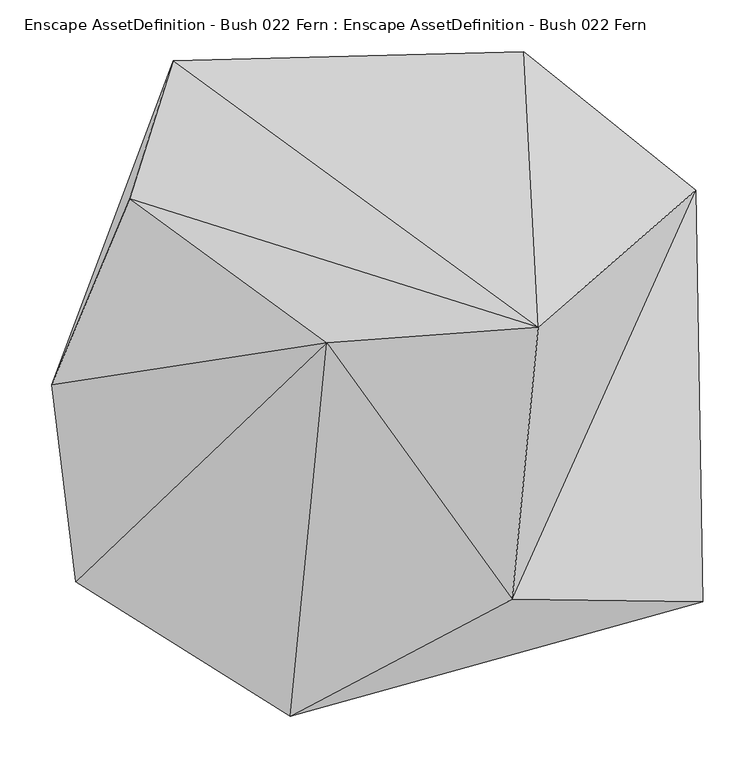
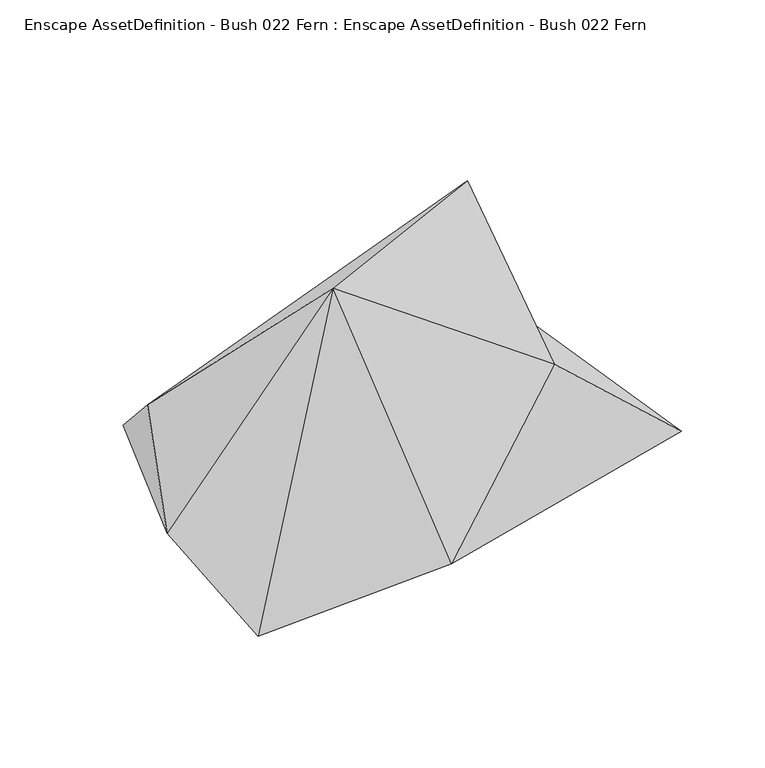
"""IFC4 building model written with IfcOpenShell, lengths in millimetres: geographic element geometry, Enscape AssetDefinition - Bush 022 Fern : Enscape AssetDefinition - Bush 022 Fern."""

from ifc_helpers import new_model, si_unit, origin, place, context, project, spatial, faceted_brep, source, transform, mapped, element, save


def enscape_assetdefinition_bush_022_fern_enscape_16470abe(model_context):
    return source(origin(), model_context, "Body", "Brep", [
        faceted_brep([(-237.1029854, 165.6155586, 164.089337), (-47.436472, 26.9630011, 361.0720038), (156.4911604, 41.8980867, 446.0159242), (-312.0678067, -13.4198414, 101.9497737), (-289.0363634, -203.1974643, 50.9199388), (131.4267814, -220.2729434, 331.5717876), (-82.5495422, -332.7048719, 168.5667038), (142.4339563, 306.9921732, 28.7053473), (308.2143664, 173.6044735, 108.4637195), (0.0, 0.0, -3.9840727), (314.9578571, -222.6221114, 165.6070352), (-195.3037977, 298.6308336, 37.6759209)], [[[0, 1, 2]], [[3, 1, 0]], [[4, 1, 3]], [[5, 1, 6]], [[2, 1, 5]], [[7, 2, 8]], [[4, 3, 9]], [[8, 5, 10]], [[2, 7, 11]], [[4, 10, 6]], [[5, 8, 2]], [[10, 9, 8]], [[8, 9, 7]], [[4, 9, 10]], [[9, 3, 11]], [[9, 11, 7]], [[6, 10, 5]], [[6, 1, 4]], [[3, 0, 11]], [[0, 2, 11]]]),
    ])


if __name__ == "__main__":
    model = new_model("IFC4")
    model_context = context("Model", 3, world=origin())
    ifc_project = project(units=[si_unit("LENGTHUNIT", "METRE", prefix="MILLI")], contexts=[model_context])
    site = spatial("IfcSite", under=ifc_project)
    building = spatial("IfcBuilding", under=site)
    placement = place(None, origin())
    enscape_assetdefinition_bush_022_fern_enscape_shape = enscape_assetdefinition_bush_022_fern_enscape_16470abe(model_context)
    element("IfcGeographicElement", 1, ObjectType="Enscape AssetDefinition - Bush 022 Fern : Enscape AssetDefinition - Bush 022 Fern", at=placement, inside=building, context=model_context, shape_type="MappedRepresentation", body=[
        mapped(enscape_assetdefinition_bush_022_fern_enscape_shape, transform((0.0, 0.0, 0.0), x_axis=(1.0, 0.0, 0.0), y_axis=(0.0, 1.0, 0.0), z_axis=(0.0, 0.0, 1.0))),
    ])
    save(model, "model.ifc")

# Revit data of these elements
# Type "Enscape AssetDefinition - Bush 022 Fern : Enscape AssetDefinition - Bush 022 Fern"
#   EnscapeAssetSource = "REMOTE"
#   EnscapeAssetId = "ca3fb51f-7cfd-4e9f-8287-cedadb532316"
#   Height = 0.446016 m
#   EnscapeNativeAssetHeight = 0.446016 m
#   Default Elevation = 0
